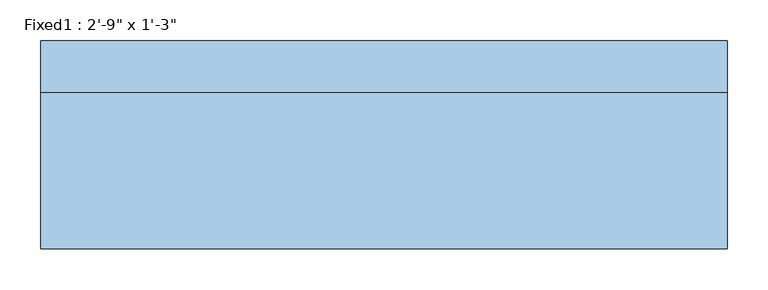
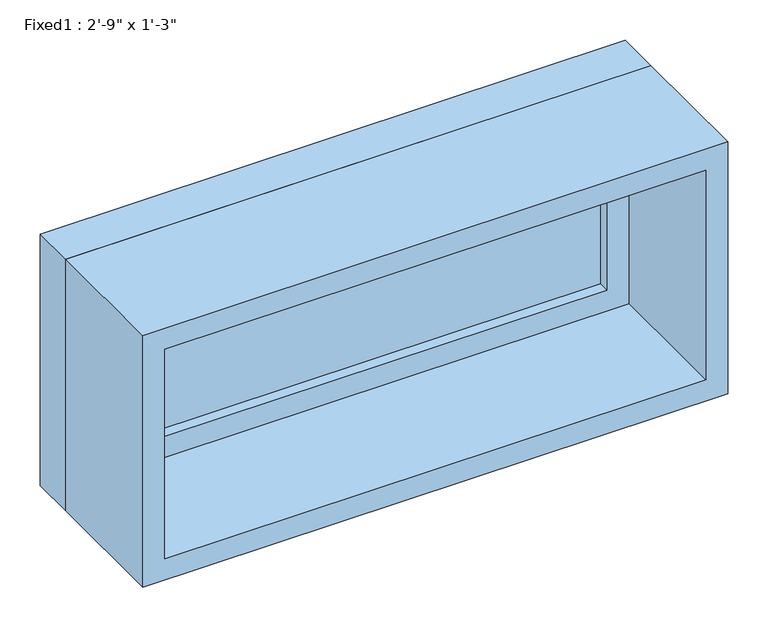
"""IFC4 building model written with IfcOpenShell, lengths in millimetres: window geometry."""

from ifc_helpers import new_model, si_unit, frame, origin, place, context, project, spatial, polyline, outline, extrude, source, transform, mapped, element, save


def window_bf5cd34b(model_context):
    return source(origin(), model_context, "Body", "SweptSolid", [
        extrude(outline(polyline([(317.5, 79.375), (-393.7, 79.375), (-393.7, 92.075), (317.5, 92.075), (317.5, 79.375)])), frame((0.0, 0.0, 977.9), z_axis=(0.0, 0.0, 1.0), x_axis=(1.0, 0.0, 0.0)), (0.0, 0.0, 1.0), 254.0),
        extrude(outline(polyline([(1276.35, -438.15), (933.45, -438.15), (933.45, 361.95), (1276.35, 361.95), (1276.35, -438.15)]), holes=[polyline([(1231.9, -393.7), (1231.9, 317.5), (977.9, 317.5), (977.9, -393.7), (1231.9, -393.7)])]), frame((0.0, 63.5, 0.0), z_axis=(0.0, 1.0, 0.0), x_axis=(0.0, 0.0, 1.0)), (0.0, 0.0, 1.0), 44.45),
        extrude(outline(polyline([(1295.4, -457.2), (914.4, -457.2), (914.4, 381.0), (1295.4, 381.0), (1295.4, -457.2)]), holes=[polyline([(1263.65, -425.45), (1263.65, 349.25), (946.15, 349.25), (946.15, -425.45), (1263.65, -425.45)])]), frame((0.0, -127.0, 0.0), z_axis=(0.0, 1.0, 0.0), x_axis=(0.0, 0.0, 1.0)), (0.0, 0.0, 1.0), 190.5),
        extrude(outline(polyline([(1295.4, 381.0), (1295.4, -457.2), (914.4, -457.2), (914.4, 381.0), (1295.4, 381.0)]), holes=[polyline([(1276.35, 361.95), (933.45, 361.95), (933.45, -438.15), (1276.35, -438.15), (1276.35, 361.95)])]), frame((0.0, 63.5, 0.0), z_axis=(0.0, 1.0, 0.0), x_axis=(0.0, 0.0, 1.0)), (0.0, 0.0, 1.0), 63.5),
    ])


if __name__ == "__main__":
    model = new_model("IFC4")
    model_context = context("Model", 3, world=origin())
    ifc_project = project(units=[si_unit("LENGTHUNIT", "METRE", prefix="MILLI")], contexts=[model_context])
    site = spatial("IfcSite", under=ifc_project)
    building = spatial("IfcBuilding", under=site)
    placement = place(None, origin())
    window_shape = window_bf5cd34b(model_context)
    element("IfcWindow", 1, ObjectType="Fixed1 : 2'-9\" x 1'-3\"", at=placement, inside=building, context=model_context, shape_type="MappedRepresentation", body=[
        mapped(window_shape, transform((0.0, 0.0, 0.0), x_axis=(1.0, 0.0, 0.0), y_axis=(0.0, 1.0, 0.0), z_axis=(0.0, 0.0, 1.0))),
    ])
    save(model, "model.ifc")

# Revit data of these elements
# Type "Fixed1 : 2'-9\" x 1'-3\""
#   Type Mark = "11"
#   Construction Type Id = "GSP4R"
#   Assembly Code = "B2020100"
#   Analytic Construction = "1/8 in Pilkington single glazing"
#   Visual Light Transmittance = 0.9
#   Solar Heat Gain Coefficient = 0.78
#   Heat Transfer Coefficient (U) = 3.6886 W/(m²·K)
#   Height = 1' - 3"
#   Default Sill Height = 3' - 0"
#   Width = 2' - 9"
#   Window Inset = 0' - 0 3/4"
#   Glass Pane Material = NEW DOUBLE HUNG WINDOWS (TYP.)
#   Sash Material = 1X WOOD COMPOSITE TRIM
#   Wall Closure = (empty or 0)
# Element 1 (IfcWindow, "Fixed1 : 2'-9\" x 1'-3\"")
#   Materials on its faces: "1X WOOD COMPOSITE TRIM", "NEW DOUBLE HUNG WINDOWS (TYP.)"
# Materials
#   "NEW DOUBLE HUNG WINDOWS (TYP.)": class "Glass", colour RGB 218 227 224, transparency 0.85, Description = "Soda Lime Glass", Cost = 0
#   "1X WOOD COMPOSITE TRIM": class "Generic", colour RGB 88 61 61, transparency 0, Cost = 0
